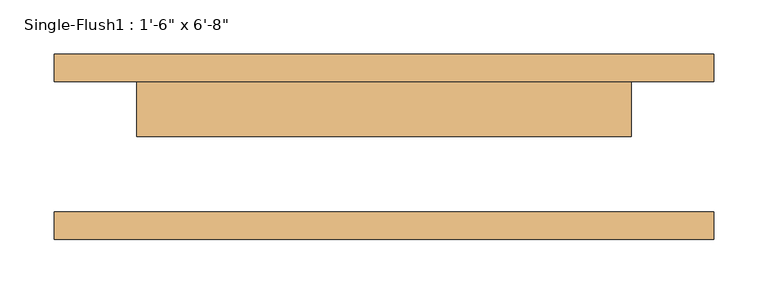
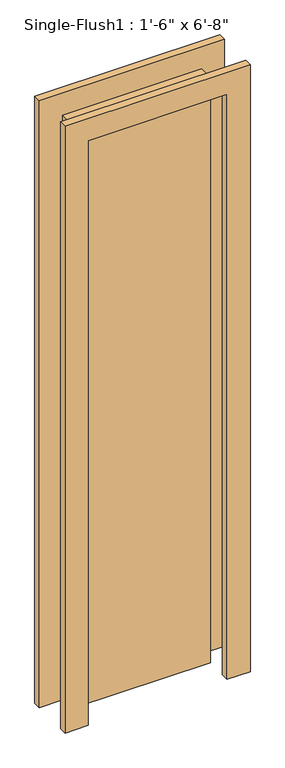
"""IFC4 building model written with IfcOpenShell, lengths in millimetres: door geometry."""

from ifc_helpers import new_model, si_unit, frame, origin, origin_with_axes, place, context, project, spatial, polyline, outline, extrude, source, transform, mapped, element, save


def door_748079e9(model_context):
    return source(origin(), model_context, "Body", "SweptSolid", [
        extrude(outline(polyline([(2108.2, -304.8), (0.0, -304.8), (0.0, -228.6), (2032.0, -228.6), (2032.0, 228.6), (0.0, 228.6), (0.0, 304.8), (2108.2, 304.8), (2108.2, -304.8)])), frame((0.0, 60.325, 0.0), z_axis=(0.0, 1.0, 0.0), x_axis=(0.0, 0.0, 1.0)), (0.0, 0.0, 1.0), 25.4),
        extrude(outline(polyline([(2108.2, 304.8), (2108.2, -304.8), (0.0, -304.8), (0.0, -228.6), (2032.0, -228.6), (2032.0, 228.6), (0.0, 228.6), (0.0, 304.8), (2108.2, 304.8)])), frame((0.0, -85.725, 0.0), z_axis=(0.0, 1.0, 0.0), x_axis=(0.0, 0.0, 1.0)), (0.0, 0.0, 1.0), 25.4),
        extrude(outline(polyline([(228.6, 9.525), (-228.6, 9.525), (-228.6, 60.325), (228.6, 60.325), (228.6, 9.525)])), origin_with_axes(), (0.0, 0.0, 1.0), 2032.0),
    ])


if __name__ == "__main__":
    model = new_model("IFC4")
    model_context = context("Model", 3, world=origin())
    ifc_project = project(units=[si_unit("LENGTHUNIT", "METRE", prefix="MILLI")], contexts=[model_context])
    site = spatial("IfcSite", under=ifc_project)
    building = spatial("IfcBuilding", under=site)
    placement = place(None, origin())
    door_shape = door_748079e9(model_context)
    element("IfcDoor", 1, ObjectType="Single-Flush1 : 1'-6\" x 6'-8\"", at=placement, inside=building, context=model_context, shape_type="MappedRepresentation", body=[
        mapped(door_shape, transform((0.0, 0.0, 0.0), x_axis=(1.0, 0.0, 0.0), y_axis=(0.0, 1.0, 0.0), z_axis=(0.0, 0.0, 1.0))),
    ])
    save(model, "model.ifc")

# Revit data of these elements
# Type "Single-Flush1 : 1'-6\" x 6'-8\""
#   Type Mark = "D5"
#   Construction Type Id = "MDOOR"
#   Assembly Code = "C1020"
#   Analytic Construction = "Metal"
#   Thickness = 0' - 2"
#   Heat Transfer Coefficient (U) = 3.7021 W/(m²·K)
#   Height = 6' - 8"
#   Trim Projection Ext = 0' - 1"
#   Trim Projection Int = 0' - 1"
#   Trim Width = 0' - 3"
#   Width = 1' - 6"
#   Door Material = Door - Panel
#   Frame Material = Door - Frame
#   Visual Light Transmittance = 0
#   Solar Heat Gain Coefficient = 0
#   Function = (empty or 0)
#   Wall Closure = (empty or 0)
# Element 1 (IfcDoor, "Single-Flush1 : 1'-6\" x 6'-8\"")
#   Materials on its faces: "Door - Frame", "Door - Panel"
# Materials
#   "Door - Panel": class "Wood", colour RGB 210 159 95, transparency 0, Cost = 0
#   "Door - Frame": class "Miscellaneous", colour RGB 118 70 51, transparency 0, Cost = 0
